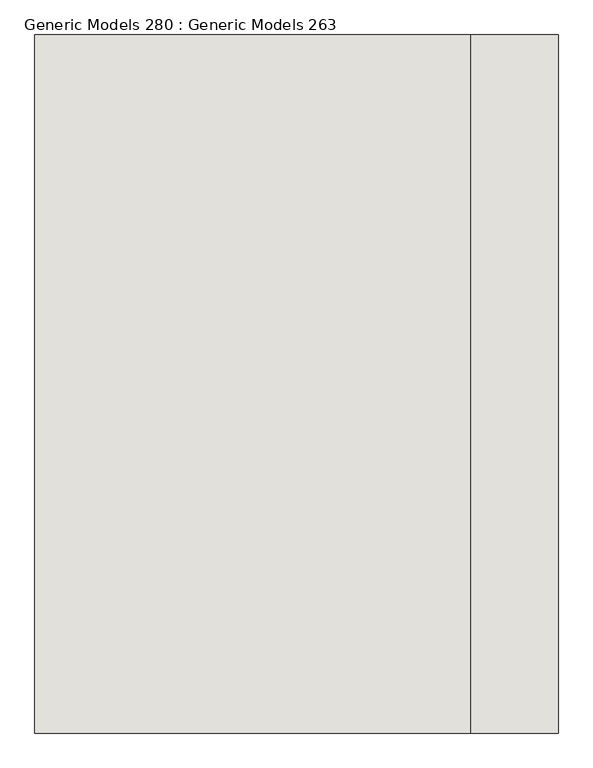
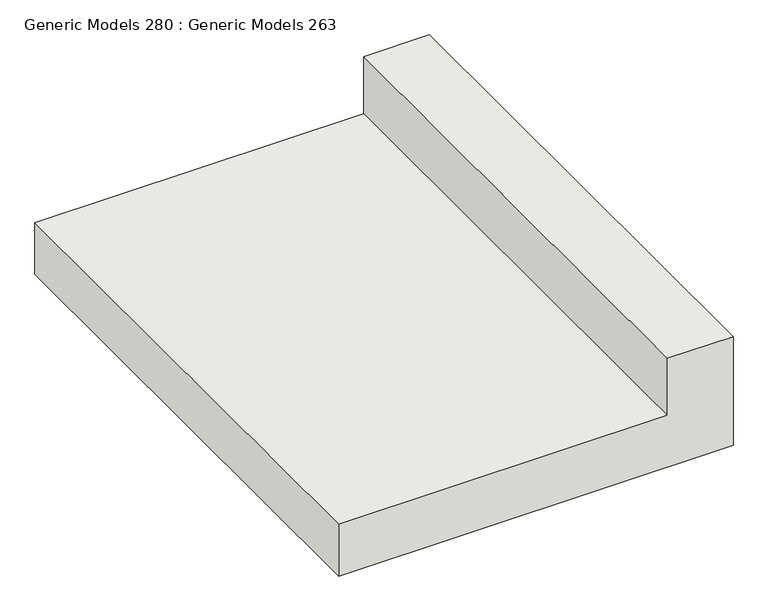
"""IFC4 building model written with IfcOpenShell, lengths in millimetres: wall geometry, Generic Models 280 : Generic Models 263."""

from ifc_helpers import new_model, si_unit, frame, origin, place, context, project, spatial, polyline, outline, extrude, source, transform, mapped, element, save


def generic_models_280_generic_models_263_4ff5fa89(model_context):
    return source(origin(), model_context, "Body", "SweptSolid", [
        extrude(outline(polyline([(-381.0, 62776.3797726), (-381.0, 62014.3797726), (-508.0, 62014.3797726), (-508.0, 62928.7797726), (-241.3, 62928.7797726), (-241.3, 62776.3797726), (-381.0, 62776.3797726)])), frame((0.0, -94.4486541, 0.0), z_axis=(0.0, 1.0, 0.0), x_axis=(0.0, 0.0, 1.0)), (0.0, 0.0, 1.0), 1219.2),
    ])


if __name__ == "__main__":
    model = new_model("IFC4")
    model_context = context("Model", 3, world=origin())
    ifc_project = project(units=[si_unit("LENGTHUNIT", "METRE", prefix="MILLI")], contexts=[model_context])
    site = spatial("IfcSite", under=ifc_project)
    building = spatial("IfcBuilding", under=site)
    placement = place(None, origin())
    generic_models_280_generic_models_263_shape = generic_models_280_generic_models_263_4ff5fa89(model_context)
    element("IfcWall", 1, ObjectType="Generic Models 280 : Generic Models 263", at=placement, inside=building, context=model_context, shape_type="MappedRepresentation", body=[
        mapped(generic_models_280_generic_models_263_shape, transform((0.0, 0.0, 0.0), x_axis=(1.0, 0.0, 0.0), y_axis=(0.0, 1.0, 0.0), z_axis=(0.0, 0.0, 1.0))),
    ])
    save(model, "model.ifc")

# Revit data of these elements
# Element 1 (IfcWall, "Generic Models 280 : Generic Models 263")
#   Materials on its faces: "5\" MIN. COMPACTED BASE AGGREGATE UNDER CURB"
# Materials
#   "5\" MIN. COMPACTED BASE AGGREGATE UNDER CURB": class "Miscellaneous", colour RGB 183 184 198, transparency 0, Cost = 0
